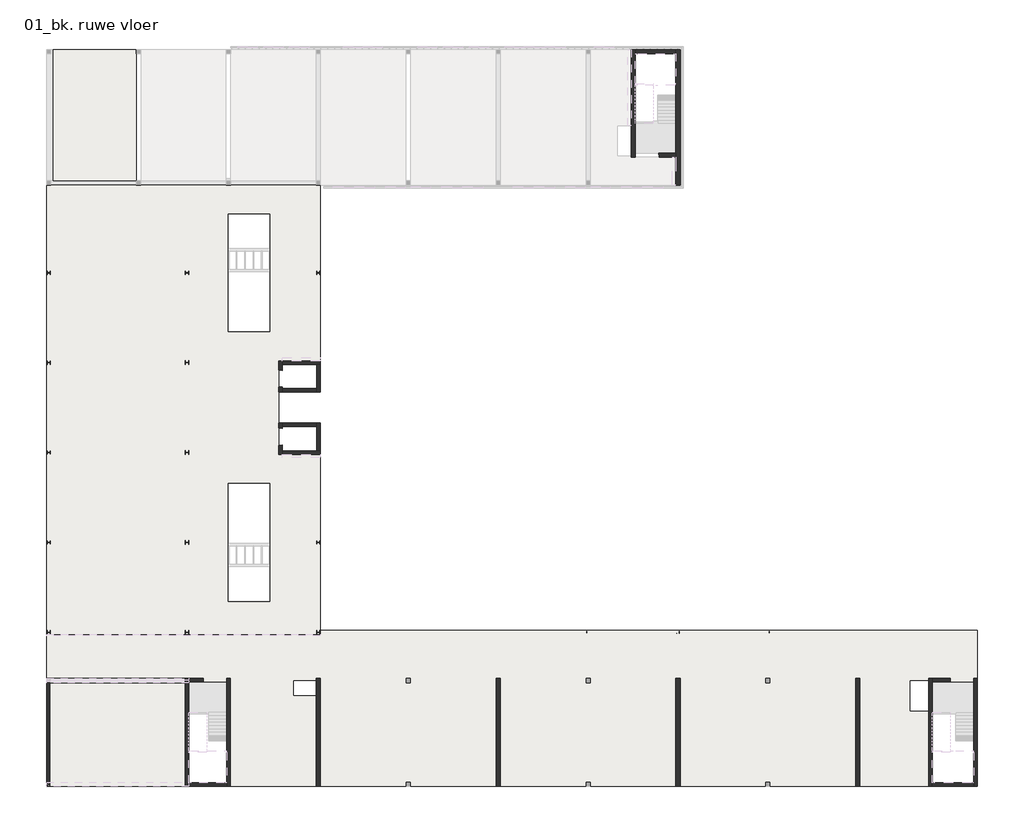
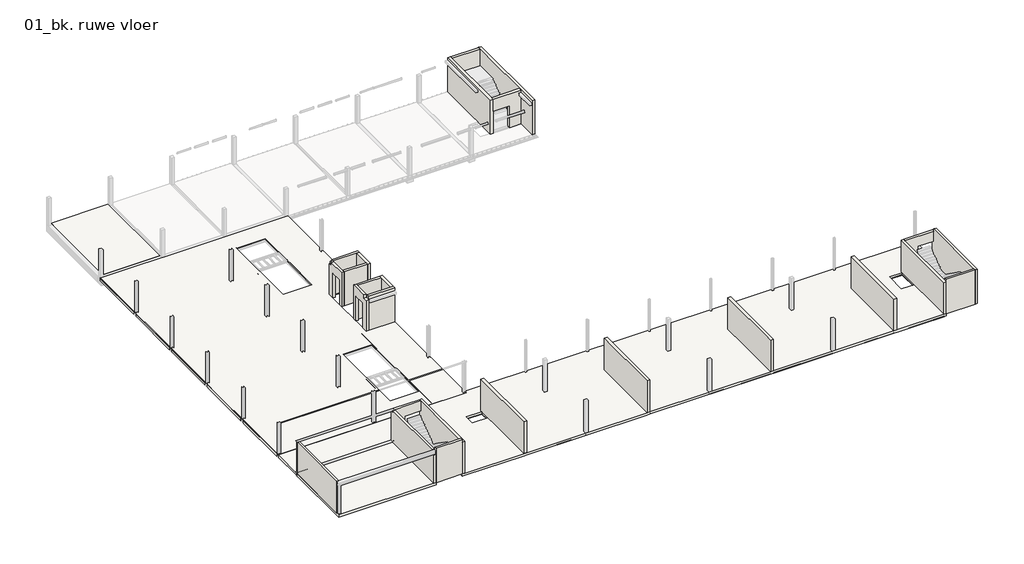
# One storey, part 1 of 4: 25 walls, 20 slabs.
"""IFC4 building model written with IfcOpenShell, lengths in millimetres."""

import ifcopenshell
import ifcopenshell.guid

model = None  # the IFC model being written
_history = None  # IfcOwnerHistory: only IFC2X3 demands one
_inside = {}  # id of a spatial element -> (the spatial element, [elements in it])
_under = {}  # id of a project, library or spatial element -> (it, [spatial elements below it])
_declared = {}  # id of a project -> (the project, [libraries it declares])
_typed = {}  # id of a type object -> (the type object, [elements of that type])
_made_of = {}  # id of a material, layer set ... -> (it, [elements and type objects made of it])


def new_model(schema):
    """Start an empty IFC model of exactly this schema.

    Asked for "IFC4X3", IfcOpenShell would pick the latest addendum, in which some entities
    have other attributes; the version numbers below select the first issue.
    IFC2X3 requires an IfcOwnerHistory on every rooted entity: one is made here for all.
    """
    global model, _history
    if schema == "IFC4X3":
        model = ifcopenshell.file(schema_version=(4, 3, 0, 0))
    else:
        model = ifcopenshell.file(schema=schema)
    _inside.clear()
    _under.clear()
    _declared.clear()
    _typed.clear()
    _made_of.clear()
    _history = None
    if model.schema == "IFC2X3":
        org = make("IfcOrganization", Name="unknown")
        user = make(
            "IfcPersonAndOrganization",
            ThePerson=make("IfcPerson", FamilyName="unknown"),
            TheOrganization=org,
        )
        app = make(
            "IfcApplication",
            ApplicationDeveloper=org,
            Version="unknown",
            ApplicationFullName="unknown",
            ApplicationIdentifier="unknown",
        )
        _history = make(
            "IfcOwnerHistory",
            OwningUser=user,
            OwningApplication=app,
            ChangeAction="ADDED",
            CreationDate=0,
        )
    return model


def make(cls, **values):
    """One entity of the class cls with the attributes given. An attribute that is None is left unset."""
    return model.create_entity(
        cls, **{name: value for name, value in values.items() if value is not None}
    )


def rooted(cls, **values):
    """An entity with a GlobalId (a new one), such as an element, a storey or a relation."""
    return make(cls, GlobalId=ifcopenshell.guid.new(), OwnerHistory=_history, **values)


def si_unit(unit_type, name, prefix=None):
    """IfcSIUnit, for example si_unit("LENGTHUNIT", "METRE", prefix="MILLI")."""
    return make("IfcSIUnit", UnitType=unit_type, Prefix=prefix, Name=name)


def assignment(units):
    """IfcUnitAssignment: the units of a project."""
    return None if units is None else make("IfcUnitAssignment", Units=units)


def point(xyz):
    """IfcCartesianPoint."""
    return None if xyz is None else make("IfcCartesianPoint", Coordinates=xyz)


def direction(xyz):
    """IfcDirection."""
    return None if xyz is None else make("IfcDirection", DirectionRatios=xyz)


def frame(location, z_axis=None, x_axis=None):
    """IfcAxis2Placement3D, a coordinate frame: its origin and axes. An axis left out is left unset."""
    return make(
        "IfcAxis2Placement3D",
        Location=point(location),
        Axis=direction(z_axis),
        RefDirection=direction(x_axis),
    )


def origin():
    """The frame at (0, 0, 0) with its axes left unset."""
    return frame((0.0, 0.0, 0.0))


def place(relative_to, where):
    """IfcLocalPlacement: puts the frame where relative to a parent placement (None: the world)."""
    return make(
        "IfcLocalPlacement", PlacementRelTo=relative_to, RelativePlacement=where
    )


def context(
    kind, dimensions, precision=None, world=None, true_north=None, identifier=None
):
    """IfcGeometricRepresentationContext, for example the 3D "Model" context."""
    return make(
        "IfcGeometricRepresentationContext",
        ContextIdentifier=identifier,
        ContextType=kind,
        CoordinateSpaceDimension=dimensions,
        Precision=precision,
        WorldCoordinateSystem=world,
        TrueNorth=true_north,
    )


def project(units=None, contexts=None):
    """IfcProject with its units and contexts."""
    return rooted(
        "IfcProject",
        Name="project",
        RepresentationContexts=contexts,
        UnitsInContext=assignment(units),
    )


def spatial(cls, under=None, at=None, **own):
    """A site, building, storey or space (cls), placed at a placement, below another one or the project."""
    s = rooted(cls, ObjectPlacement=at, **own)
    if under is not None:
        _under.setdefault(under.id(), (under, []))[1].append(s)
    return s


def polyline(points):
    """IfcPolyline through the points."""
    return make("IfcPolyline", Points=[point(p) for p in points])


def outline(outer, holes=None, kind="AREA"):
    """IfcArbitraryClosedProfileDef: a profile drawn as a closed curve; with holes, ...WithVoids."""
    if holes is None:
        return make("IfcArbitraryClosedProfileDef", ProfileType=kind, OuterCurve=outer)
    return make(
        "IfcArbitraryProfileDefWithVoids",
        ProfileType=kind,
        OuterCurve=outer,
        InnerCurves=holes,
    )


def extrude(swept, where, along, depth):
    """IfcExtrudedAreaSolid: the profile swept, set in the frame where, extruded along a direction by depth."""
    return make(
        "IfcExtrudedAreaSolid",
        SweptArea=swept,
        Position=where,
        ExtrudedDirection=direction(along),
        Depth=depth,
    )


def faces_of(points, faces, orient=None, outer=None):
    """IfcFace entities. A face is a list of loops; a loop is a list of indices into points, from 0.

    orient and outer hold one flag for each loop. By default every Orientation is true, the
    first loop of a face is its IfcFaceOuterBound and the others are IfcFaceBound.
    """
    made = []
    for i, loops in enumerate(faces):
        bounds = []
        for j, loop in enumerate(loops):
            is_outer = j == 0 if outer is None else outer[i][j]
            bounds.append(
                make(
                    "IfcFaceOuterBound" if is_outer else "IfcFaceBound",
                    Bound=make("IfcPolyLoop", Polygon=[points[k] for k in loop]),
                    Orientation=True if orient is None else orient[i][j],
                )
            )
        made.append(make("IfcFace", Bounds=bounds))
    return made


def faceted_brep(points, faces, orient=None, outer=None, voids=None):
    """IfcFacetedBrep: a solid bounded by flat faces; with voids (closed shells), ...WithVoids."""
    shared = [point(p) for p in points]
    hull = make("IfcClosedShell", CfsFaces=faces_of(shared, faces, orient, outer))
    if voids is None:
        return make("IfcFacetedBrep", Outer=hull)
    return make(
        "IfcFacetedBrepWithVoids",
        Outer=hull,
        Voids=[
            make(cls, CfsFaces=faces_of(shared, fs, o, b)) for cls, fs, o, b in voids
        ],
    )


def shape(context_of_items, identifier, shape_type, items):
    """IfcShapeRepresentation: the items that make up one representation, for example the "Body"."""
    return make(
        "IfcShapeRepresentation",
        ContextOfItems=context_of_items,
        RepresentationIdentifier=identifier,
        RepresentationType=shape_type,
        Items=items,
    )


def made_of(thing, what):
    """Note that an element or type object is made of a material, layer set ...; save() writes the relation."""
    if what is not None:
        _made_of.setdefault(what.id(), (what, []))[1].append(thing)
    return thing


def element(
    cls,
    number,
    at=None,
    inside=None,
    cuts=None,
    type_object=None,
    material=None,
    context=None,
    identifier="Body",
    shape_type=None,
    held_by="IfcProductDefinitionShape",
    body=None,
    shapes=None,
    **own,
):
    """One element of the class cls, such as IfcWall. Its Tag is "e" and its number.

    at: its placement. inside: the storey or other place that contains it. cuts: it is an
    opening in that element (IfcRelVoidsElement). A single representation is given by context,
    identifier, shape_type and body (its items); several are given by shapes. held_by: the class
    of the entity that holds the representations. save() writes the other relations.
    """
    e = rooted(cls, Tag="e%d" % number, ObjectPlacement=at, **own)
    if body is not None:
        shapes = [shape(context, identifier, shape_type, body)]
    if shapes is not None:
        e.Representation = make(held_by, Representations=shapes)
    if inside is not None:
        _inside.setdefault(inside.id(), (inside, []))[1].append(e)
    if cuts is not None:
        rooted(
            "IfcRelVoidsElement", RelatingBuildingElement=cuts, RelatedOpeningElement=e
        )
    if type_object is not None:
        _typed.setdefault(type_object.id(), (type_object, []))[1].append(e)
    return made_of(e, material)


def aggregate(whole, parts):
    """IfcRelAggregates: a whole, such as a stair, and the parts it consists of."""
    return rooted("IfcRelAggregates", RelatingObject=whole, RelatedObjects=parts)


def save(model, path):
    """Write the relations noted so far, then the file.

    IfcRelAggregates (storeys below a building ...), IfcRelContainedInSpatialStructure (elements
    in a storey), IfcRelDefinesByType, IfcRelAssociatesMaterial and IfcRelDeclares: one each for
    every whole, place, type object, material and project.
    """
    for whole, parts in _under.values():
        aggregate(whole, parts)
    for where, things in _inside.values():
        rooted(
            "IfcRelContainedInSpatialStructure",
            RelatedElements=things,
            RelatingStructure=where,
        )
    for kind, things in _typed.values():
        rooted("IfcRelDefinesByType", RelatedObjects=things, RelatingType=kind)
    for what, things in _made_of.values():
        rooted("IfcRelAssociatesMaterial", RelatedObjects=things, RelatingMaterial=what)
    for by, libraries in _declared.values():
        rooted("IfcRelDeclares", RelatingContext=by, RelatedDefinitions=libraries)
    model.write(path)


model = new_model("IFC4")

# Units and contexts
model_context = context("Model", 3, world=origin())
ifc_project = project(units=[si_unit("LENGTHUNIT", "METRE", prefix="MILLI")], contexts=[model_context])

# Site, building, storey
site = spatial("IfcSite", under=ifc_project)
building = spatial("IfcBuilding", under=site)
storey = spatial("IfcBuildingStorey", under=building, Name="01_bk. ruwe vloer", Elevation=3730.0)

# Slabs
placement = place(None, origin())
element("IfcSlab", 1, ObjectType="NLRS_23_FL_breedplaat 260_gen_rsf", at=placement, inside=storey, context=model_context, shape_type="Brep", body=[
    faceted_brep([(70375.0, -150.0, 3470.0), (70125.0, -150.0, 3470.0), (65200.0, -150.0, 3470.0), (64800.0, -150.0, 3470.0), (52200.0, -150.0, 3470.0), (51800.0, -150.0, 3470.0), (39200.0, -150.0, 3470.0), (38800.0, -150.0, 3470.0), (26200.0, -150.0, 3470.0), (25800.0, -150.0, 3470.0), (19625.0, -150.0, 3470.0), (19375.0, -150.0, 3470.0), (19375.0, 7400.0, 3470.0), (16625.0, 7400.0, 3470.0), (16625.0, 7493.0, 3470.0), (16625.0, 7507.0, 3470.0), (6350.0, 7507.0, 3470.0), (6350.0, 10845.0, 3470.0), (26125.0, 10845.0, 3470.0), (26125.0, 11125.0, 3470.0), (73650.0, 11125.0, 3470.0), (73650.0, 7400.0, 3470.0), (73400.0, 7400.0, 3470.0), (70375.0, 7400.0, 3470.0), (19600.0, 7622.0, 3470.0), (19600.0, -140.0, 3470.0), (25825.0, -140.0, 3470.0), (25825.0, 125.0, 3470.0), (26175.0, 125.0, 3470.0), (26175.0, -140.0, 3470.0), (32375.0, -140.0, 3470.0), (32375.0, 7625.0, 3470.0), (32625.0, 7625.0, 3470.0), (32625.0, -140.0, 3470.0), (38825.0, -140.0, 3470.0), (38825.0, 125.0, 3470.0), (39175.0, 125.0, 3470.0), (39175.0, -140.0, 3470.0), (45375.0, -140.0, 3470.0), (45375.0, 7625.0, 3470.0), (45625.0, 7625.0, 3470.0), (45625.0, -140.0, 3470.0), (51825.0, -140.0, 3470.0), (51825.0, 125.0, 3470.0), (52175.0, 125.0, 3470.0), (52175.0, -140.0, 3470.0), (58375.0, -140.0, 3470.0), (58375.0, 7625.0, 3470.0), (58625.0, 7625.0, 3470.0), (58625.0, -140.0, 3470.0), (64825.0, -140.0, 3470.0), (64825.0, 125.0, 3470.0), (65175.0, 125.0, 3470.0), (65175.0, -140.0, 3470.0), (70150.0, -140.0, 3470.0), (70150.0, 7625.0, 3470.0), (73640.0, 7625.0, 3470.0), (73640.0, 11115.0, 3470.0), (26135.0, 11115.0, 3470.0), (26135.0, 10750.0, 3470.0), (6360.0, 10750.0, 3470.0), (6360.0, 7622.0, 3470.0), (51825.0, 7625.0, 3470.0), (52175.0, 7625.0, 3470.0), (52175.0, 7375.0, 3470.0), (51825.0, 7375.0, 3470.0), (64825.0, 7625.0, 3470.0), (65175.0, 7625.0, 3470.0), (65175.0, 7375.0, 3470.0), (64825.0, 7375.0, 3470.0), (38825.0, 7625.0, 3470.0), (39175.0, 7625.0, 3470.0), (39175.0, 7375.0, 3470.0), (38825.0, 7375.0, 3470.0), (25850.0, 7375.0, 3470.0), (25850.0, 7500.0, 3470.0), (25825.0, 7500.0, 3470.0), (25825.0, 7625.0, 3470.0), (26175.0, 7625.0, 3470.0), (26175.0, 7375.0, 3470.0), (19375.0, -150.0, 3730.0), (19625.0, -150.0, 3730.0), (25850.0, -150.0, 3730.0), (26150.0, -150.0, 3730.0), (32350.0, -150.0, 3730.0), (32650.0, -150.0, 3730.0), (38850.0, -150.0, 3730.0), (39150.0, -150.0, 3730.0), (45350.0, -150.0, 3730.0), (45650.0, -150.0, 3730.0), (51850.0, -150.0, 3730.0), (52150.0, -150.0, 3730.0), (58350.0, -150.0, 3730.0), (58650.0, -150.0, 3730.0), (64850.0, -150.0, 3730.0), (65150.0, -150.0, 3730.0), (70125.0, -150.0, 3730.0), (70375.0, -150.0, 3730.0), (70375.0, 7400.0, 3730.0), (71700.0, 7400.0, 3730.0), (73650.0, 7400.0, 3730.0), (73650.0, 11125.0, 3730.0), (26125.0, 11125.0, 3730.0), (26125.0, 10845.0, 3730.0), (6350.0, 10845.0, 3730.0), (6350.0, 7507.0, 3730.0), (16625.0, 7507.0, 3730.0), (16625.0, 7493.0, 3730.0), (16625.0, 7400.0, 3730.0), (19375.0, 7400.0, 3730.0), (19375.0, 100.0, 3730.0), (24227.5, 6452.0, 3730.0), (24227.5, 7500.0, 3730.0), (25850.0, 7500.0, 3730.0), (25850.0, 6452.0, 3730.0), (68805.0, 5320.0, 3730.0), (68805.0, 7500.0, 3730.0), (70125.0, 7500.0, 3730.0), (70125.0, 5320.0, 3730.0), (6350.0, 10845.0, 3680.0), (26125.0, 10845.0, 3680.0), (19600.0, -140.0, 3530.0), (19600.0, 7622.0, 3530.0), (6360.0, 7622.0, 3530.0), (6360.0, 10750.0, 3530.0), (26135.0, 10750.0, 3530.0), (26135.0, 11115.0, 3530.0), (73640.0, 11115.0, 3530.0), (73640.0, 7625.0, 3530.0), (70150.0, 7625.0, 3530.0), (70150.0, -140.0, 3530.0), (65175.0, -140.0, 3530.0), (65175.0, 125.0, 3530.0), (64825.0, 125.0, 3530.0), (64825.0, -140.0, 3530.0), (58625.0, -140.0, 3530.0), (58625.0, 7625.0, 3530.0), (58375.0, 7625.0, 3530.0), (58375.0, -140.0, 3530.0), (52175.0, -140.0, 3530.0), (52175.0, 125.0, 3530.0), (51825.0, 125.0, 3530.0), (51825.0, -140.0, 3530.0), (45625.0, -140.0, 3530.0), (45625.0, 7625.0, 3530.0), (45375.0, 7625.0, 3530.0), (45375.0, -140.0, 3530.0), (39175.0, -140.0, 3530.0), (39175.0, 125.0, 3530.0), (38825.0, 125.0, 3530.0), (38825.0, -140.0, 3530.0), (32625.0, -140.0, 3530.0), (32625.0, 7625.0, 3530.0), (32375.0, 7625.0, 3530.0), (32375.0, -140.0, 3530.0), (26175.0, -140.0, 3530.0), (26175.0, 125.0, 3530.0), (25825.0, 125.0, 3530.0), (25825.0, -140.0, 3530.0), (26175.0, 7625.0, 3530.0), (25825.0, 7625.0, 3530.0), (25825.0, 7500.0, 3530.0), (24227.5, 7500.0, 3530.0), (24227.5, 6452.0, 3530.0), (25850.0, 6452.0, 3530.0), (25850.0, 7375.0, 3530.0), (26175.0, 7375.0, 3530.0), (52175.0, 7625.0, 3530.0), (51825.0, 7625.0, 3530.0), (51825.0, 7375.0, 3530.0), (52175.0, 7375.0, 3530.0), (65175.0, 7625.0, 3530.0), (64825.0, 7625.0, 3530.0), (64825.0, 7375.0, 3530.0), (65175.0, 7375.0, 3530.0), (39175.0, 7625.0, 3530.0), (38825.0, 7625.0, 3530.0), (38825.0, 7375.0, 3530.0), (39175.0, 7375.0, 3530.0), (68805.0, 7500.0, 3530.0), (68805.0, 5320.0, 3530.0), (70125.0, 5320.0, 3530.0), (70125.0, 7500.0, 3530.0)], [[[0, 1, 2, 3, 4, 5, 6, 7, 8, 9, 10, 11, 12, 13, 14, 15, 16, 17, 18, 19, 20, 21, 22, 23], [24, 25, 26, 27, 28, 29, 30, 31, 32, 33, 34, 35, 36, 37, 38, 39, 40, 41, 42, 43, 44, 45, 46, 47, 48, 49, 50, 51, 52, 53, 54, 55, 56, 57, 58, 59, 60, 61]], [[62, 63, 64, 65]], [[66, 67, 68, 69]], [[70, 71, 72, 73]], [[74, 75, 76, 77, 78, 79]], [[80, 81, 82, 83, 84, 85, 86, 87, 88, 89, 90, 91, 92, 93, 94, 95, 96, 97, 98, 99, 100, 101, 102, 103, 104, 105, 106, 107, 108, 109, 110], [111, 112, 113, 114], [115, 116, 117, 118]], [[11, 10, 9, 8, 7, 6, 5, 4, 3, 2, 1, 0, 97, 96, 95, 94, 93, 92, 91, 90, 89, 88, 87, 86, 85, 84, 83, 82, 81, 80]], [[12, 11, 80, 110, 109]], [[13, 12, 109, 108]], [[13, 108, 107, 106, 15, 14]], [[17, 16, 105, 104, 119]], [[18, 17, 119, 104, 103, 120]], [[19, 18, 120, 103, 102]], [[20, 19, 102, 101]], [[21, 20, 101, 100]], [[23, 22, 21, 100, 99, 98]], [[0, 23, 98, 97]], [[16, 15, 106, 105]], [[121, 122, 123, 124, 125, 126, 127, 128, 129, 130, 131, 132, 133, 134, 135, 136, 137, 138, 139, 140, 141, 142, 143, 144, 145, 146, 147, 148, 149, 150, 151, 152, 153, 154, 155, 156, 157, 158], [159, 160, 161, 162, 163, 164, 165, 166], [167, 168, 169, 170], [171, 172, 173, 174], [175, 176, 177, 178], [179, 180, 181, 182]], [[122, 121, 25, 24]], [[123, 122, 24, 61]], [[124, 123, 61, 60]], [[125, 124, 60, 59]], [[126, 125, 59, 58]], [[127, 126, 58, 57]], [[128, 127, 57, 56]], [[129, 128, 56, 55]], [[130, 129, 55, 54]], [[131, 130, 54, 53]], [[132, 131, 53, 52]], [[133, 132, 52, 51]], [[134, 133, 51, 50]], [[135, 134, 50, 49]], [[136, 135, 49, 48]], [[137, 136, 48, 47]], [[138, 137, 47, 46]], [[139, 138, 46, 45]], [[140, 139, 45, 44]], [[141, 140, 44, 43]], [[142, 141, 43, 42]], [[143, 142, 42, 41]], [[144, 143, 41, 40]], [[145, 144, 40, 39]], [[146, 145, 39, 38]], [[147, 146, 38, 37]], [[148, 147, 37, 36]], [[149, 148, 36, 35]], [[150, 149, 35, 34]], [[151, 150, 34, 33]], [[152, 151, 33, 32]], [[153, 152, 32, 31]], [[154, 153, 31, 30]], [[155, 154, 30, 29]], [[156, 155, 29, 28]], [[157, 156, 28, 27]], [[158, 157, 27, 26]], [[121, 158, 26, 25]], [[160, 159, 78, 77]], [[161, 160, 77, 76]], [[166, 165, 74, 79]], [[159, 166, 79, 78]], [[168, 167, 63, 62]], [[169, 168, 62, 65]], [[170, 169, 65, 64]], [[167, 170, 64, 63]], [[172, 171, 67, 66]], [[173, 172, 66, 69]], [[174, 173, 69, 68]], [[171, 174, 68, 67]], [[176, 175, 71, 70]], [[177, 176, 70, 73]], [[178, 177, 73, 72]], [[175, 178, 72, 71]], [[112, 111, 163, 162]], [[111, 114, 164, 163]], [[113, 75, 74, 165, 164, 114]], [[75, 113, 112, 162, 161, 76]], [[116, 115, 180, 179]], [[115, 118, 181, 180]], [[118, 117, 182, 181]], [[117, 116, 179, 182]]]),
])
element("IfcSlab", 2, ObjectType="NLRS_23_FL_breedplaat 260_gen_rsf", at=placement, inside=storey, context=model_context, shape_type="Brep", body=[
    faceted_brep([(6830.0, 43680.0, 3470.0), (6830.0, 43800.0, 3470.0), (6830.0, 53150.0, 3470.0), (6950.0, 53150.0, 3470.0), (12700.0, 53150.0, 3470.0), (12820.0, 53150.0, 3470.0), (12820.0, 43680.0, 3470.0), (12700.0, 43680.0, 3470.0), (12725.0, 43775.0, 3470.0), (12725.0, 53140.0, 3470.0), (6925.0, 53140.0, 3470.0), (6925.0, 43775.0, 3470.0), (6830.0, 53150.0, 3730.0), (6830.0, 43680.0, 3730.0), (12820.0, 43680.0, 3730.0), (12820.0, 53150.0, 3730.0), (6925.0, 53140.0, 3530.0), (12725.0, 53140.0, 3530.0), (12725.0, 43775.0, 3530.0), (6925.0, 43775.0, 3530.0)], [[[0, 1, 2, 3, 4, 5, 6, 7], [8, 9, 10, 11]], [[12, 13, 14, 15]], [[2, 1, 0, 13, 12]], [[5, 4, 3, 2, 12, 15]], [[6, 5, 15, 14]], [[0, 7, 6, 14, 13]], [[16, 17, 18, 19]], [[18, 17, 9, 8]], [[19, 18, 8, 11]], [[16, 19, 11, 10]], [[17, 16, 10, 9]]]),
])
element("IfcSlab", 3, ObjectType="NLRS_23_FL_druklaag 70_gen_rsf", at=placement, inside=storey, context=model_context, shape_type="Brep", body=[
    faceted_brep([(26125.0, 23875.0, 3660.0), (26125.0, 23795.0, 3660.0), (26125.0, 17675.0, 3660.0), (26125.0, 17655.0, 3660.0), (26125.0, 17345.0, 3660.0), (26125.0, 17325.0, 3660.0), (26125.0, 11175.0, 3660.0), (26125.0, 11155.0, 3660.0), (6350.0, 11155.0, 3660.0), (6350.0, 11175.0, 3660.0), (6350.0, 17325.0, 3660.0), (6350.0, 17345.0, 3660.0), (19240.0, 17345.0, 3660.0), (19240.0, 17655.0, 3660.0), (6350.0, 17655.0, 3660.0), (6350.0, 17675.0, 3660.0), (6350.0, 23825.0, 3660.0), (6350.0, 23845.0, 3660.0), (19240.0, 23845.0, 3660.0), (19500.0, 23845.0, 3660.0), (22500.0, 23845.0, 3660.0), (22760.0, 23845.0, 3660.0), (23362.3, 23845.0, 3660.0), (23362.3, 23875.0, 3660.0), (22500.0, 21750.0, 3660.0), (19500.0, 21750.0, 3660.0), (19500.0, 13250.0, 3660.0), (22500.0, 13250.0, 3660.0), (19500.0000006, 22062.0, 3660.0), (19500.0000006, 21760.0, 3660.0), (22499.9999994, 21760.0, 3660.0), (22499.9999994, 22062.0, 3660.0), (19500.0000006, 13240.0, 3660.0), (19500.0000006, 12938.0, 3660.0), (22499.9999994, 12938.0, 3660.0), (22499.9999994, 13240.0, 3660.0), (23125.0, 24155.0, 3660.0), (6350.0, 24155.0, 3660.0), (6350.0, 24175.0, 3660.0), (6350.0, 30302.0, 3660.0), (6350.0, 30322.0, 3660.0), (23125.0, 30322.0, 3660.0), (23125.0, 30302.0, 3660.0), (23125.0, 24175.0, 3660.0), (6350.0, 43350.0, 3660.0), (26125.0, 43350.0, 3660.0), (26125.0, 43330.0, 3660.0), (26125.0, 37175.0, 3660.0), (26125.0, 37155.0, 3660.0), (22760.0, 37155.0, 3660.0), (22760.0, 36845.0, 3660.0), (26125.0, 36845.0, 3660.0), (26125.0, 36825.0, 3660.0), (26125.0, 30705.0, 3660.0), (26125.0, 30625.0, 3660.0), (23362.3, 30625.0, 3660.0), (23362.3, 30632.0, 3660.0), (6350.0, 30632.0, 3660.0), (6350.0, 30652.0, 3660.0), (6350.0, 36825.0, 3660.0), (6350.0, 36845.0, 3660.0), (19240.0, 36845.0, 3660.0), (19240.0, 37155.0, 3660.0), (6350.0, 37155.0, 3660.0), (6350.0, 37175.0, 3660.0), (6350.0, 43330.0, 3660.0), (22500.0, 32750.0, 3660.0), (22500.0, 41250.0, 3660.0), (19500.0, 41250.0, 3660.0), (19500.0, 32750.0, 3660.0), (19500.0000006, 41562.0, 3660.0), (19500.0000006, 41260.0, 3660.0), (22499.9999994, 41260.0, 3660.0), (22499.9999994, 41562.0, 3660.0), (19500.0000006, 32740.0, 3660.0), (19500.0000006, 32438.0, 3660.0), (22499.9999994, 32438.0, 3660.0), (22499.9999994, 32740.0, 3660.0), (26125.0, 30625.0, 3730.0), (26125.0, 43350.0, 3730.0), (13180.0, 43350.0, 3730.0), (12820.0, 43350.0, 3730.0), (6350.0, 43350.0, 3730.0), (6350.0, 10845.0, 3730.0), (26125.0, 10845.0, 3730.0), (26125.0, 11125.0, 3730.0), (26125.0, 23875.0, 3730.0), (23125.0, 23875.0, 3730.0), (23125.0, 30625.0, 3730.0), (22500.0, 41250.0, 3730.0), (22500.0, 32750.0, 3730.0), (19500.0, 32750.0, 3730.0), (19500.0, 41250.0, 3730.0), (19500.0, 21750.0, 3730.0), (22500.0, 21750.0, 3730.0), (22500.0, 13250.0, 3730.0), (19500.0, 13250.0, 3730.0), (26125.0, 36845.0, 3680.0), (26125.0, 37155.0, 3680.0), (6350.0, 10845.0, 3680.0), (26125.0, 10845.0, 3680.0), (6350.0, 37155.0, 3680.0), (6350.0, 36845.0, 3680.0), (6350.0, 30632.0, 3680.0), (6350.0, 30322.0, 3680.0), (6350.0, 24155.0, 3680.0), (6350.0, 23845.0, 3680.0), (6350.0, 17655.0, 3680.0), (6350.0, 17345.0, 3680.0), (6350.0, 11155.0, 3680.0), (23125.0, 30625.0, 3680.0), (23362.3, 30625.0, 3680.0), (23125.0, 23875.0, 3680.0), (23125.0, 24155.0, 3680.0), (23125.0, 30322.0, 3680.0), (23362.3, 23875.0, 3680.0), (26125.0, 11125.0, 3680.0), (26125.0, 11155.0, 3680.0), (19240.0, 17345.0, 3680.0), (19240.0, 17655.0, 3680.0), (23362.3, 23845.0, 3680.0), (23362.3, 30632.0, 3680.0), (19240.0, 36845.0, 3680.0), (19240.0, 37155.0, 3680.0), (22760.0, 37155.0, 3680.0), (22760.0, 36845.0, 3680.0), (19500.0000006, 41562.0, 3680.0), (19500.0000006, 41260.0, 3680.0), (22499.9999994, 41260.0, 3680.0), (22499.9999994, 41562.0, 3680.0), (19500.0000006, 32740.0, 3680.0), (19500.0000006, 32438.0, 3680.0), (22499.9999994, 32438.0, 3680.0), (22499.9999994, 32740.0, 3680.0), (19500.0000006, 22062.0, 3680.0), (19500.0000006, 21760.0, 3680.0), (22499.9999994, 21760.0, 3680.0), (22499.9999994, 22062.0, 3680.0), (19500.0000006, 13240.0, 3680.0), (19500.0000006, 12938.0, 3680.0), (22499.9999994, 12938.0, 3680.0), (22499.9999994, 13240.0, 3680.0)], [[[0, 1, 2, 3, 4, 5, 6, 7, 8, 9, 10, 11, 12, 13, 14, 15, 16, 17, 18, 19, 20, 21, 22, 23], [24, 25, 26, 27], [28, 29, 30, 31], [32, 33, 34, 35]], [[36, 37, 38, 39, 40, 41, 42, 43]], [[44, 45, 46, 47, 48, 49, 50, 51, 52, 53, 54, 55, 56, 57, 58, 59, 60, 61, 62, 63, 64, 65], [66, 67, 68, 69], [70, 71, 72, 73], [74, 75, 76, 77]], [[78, 79, 80, 81, 82, 83, 84, 85, 86, 87, 88], [89, 90, 91, 92], [93, 94, 95, 96]], [[79, 78, 54, 53, 52, 51, 97, 98, 48, 47, 46, 45]], [[84, 83, 99, 100]], [[83, 82, 44, 65, 64, 63, 101, 102, 60, 59, 58, 57, 103, 104, 40, 39, 38, 37, 105, 106, 17, 16, 15, 14, 107, 108, 11, 10, 9, 8, 109, 99]], [[45, 44, 82, 81, 80, 79]], [[78, 88, 110, 111, 55, 54]], [[88, 87, 112, 113, 36, 43, 42, 41, 114, 110]], [[87, 86, 0, 23, 115, 112]], [[0, 86, 85, 84, 100, 116, 117, 7, 6, 5, 4, 3, 2, 1]], [[67, 66, 90, 89]], [[68, 67, 89, 92]], [[69, 68, 92, 91]], [[66, 69, 91, 90]], [[25, 24, 94, 93]], [[26, 25, 93, 96]], [[27, 26, 96, 95]], [[24, 27, 95, 94]], [[109, 117, 116, 100, 99]], [[117, 109, 8, 7]], [[118, 119, 13, 12]], [[119, 118, 108, 107]], [[119, 107, 14, 13]], [[108, 118, 12, 11]], [[120, 115, 23, 22]], [[120, 106, 105, 113, 112, 115]], [[113, 105, 37, 36]], [[106, 120, 22, 21, 20, 19, 18, 17]], [[111, 121, 56, 55]], [[103, 121, 111, 110, 114, 104]], [[121, 103, 57, 56]], [[104, 114, 41, 40]], [[122, 123, 62, 61]], [[123, 122, 102, 101]], [[123, 101, 63, 62]], [[102, 122, 61, 60]], [[124, 125, 50, 49]], [[125, 124, 98, 97]], [[98, 124, 49, 48]], [[125, 97, 51, 50]], [[126, 127, 71, 70]], [[128, 129, 73, 72]], [[127, 126, 129, 128]], [[127, 128, 72, 71]], [[129, 126, 70, 73]], [[130, 131, 75, 74]], [[132, 133, 77, 76]], [[131, 130, 133, 132]], [[133, 130, 74, 77]], [[131, 132, 76, 75]], [[134, 135, 29, 28]], [[136, 137, 31, 30]], [[135, 134, 137, 136]], [[135, 136, 30, 29]], [[137, 134, 28, 31]], [[138, 139, 33, 32]], [[140, 141, 35, 34]], [[139, 138, 141, 140]], [[141, 138, 32, 35]], [[139, 140, 34, 33]]]),
])
element("IfcSlab", 4, ObjectType="NLRS_23_FL_kanaalplaat 260_gen_rsf", at=placement, inside=storey, context=model_context, shape_type="SweptSolid", body=[
    extrude(outline(polyline([(19240.0, 11175.0), (6350.0, 11175.0), (6350.0, 17325.0), (19240.0, 17325.0), (19240.0, 11175.0)])), frame((0.0, 0.0, 3400.0), z_axis=(0.0, 0.0, 1.0), x_axis=(1.0, 0.0, 0.0)), (0.0, 0.0, 1.0), 260.0),
])
element("IfcSlab", 5, ObjectType="NLRS_23_FL_kanaalplaat 260_gen_rsf", at=placement, inside=storey, context=model_context, shape_type="SweptSolid", body=[
    extrude(outline(polyline([(6350.0, 17675.0), (6350.0, 23825.0), (19240.0, 23825.0), (19240.0, 17675.0), (6350.0, 17675.0)])), frame((0.0, 0.0, 3400.0), z_axis=(0.0, 0.0, 1.0), x_axis=(1.0, 0.0, 0.0)), (0.0, 0.0, 1.0), 260.0),
])
element("IfcSlab", 6, ObjectType="NLRS_23_FL_kanaalplaat 260_gen_rsf", at=placement, inside=storey, context=model_context, shape_type="SweptSolid", body=[
    extrude(outline(polyline([(23125.0, 30302.0), (23125.0, 24175.0), (6350.0, 24175.0), (6350.0, 30302.0), (23125.0, 30302.0)])), frame((0.0, 0.0, 3400.0), z_axis=(0.0, 0.0, 1.0), x_axis=(1.0, 0.0, 0.0)), (0.0, 0.0, 1.0), 260.0),
])
element("IfcSlab", 7, ObjectType="NLRS_23_FL_kanaalplaat 260_gen_rsf", at=placement, inside=storey, context=model_context, shape_type="SweptSolid", body=[
    extrude(outline(polyline([(22500.0, 23825.0), (22500.0, 22082.0), (19500.0, 22082.0), (19500.0, 23825.0), (22500.0, 23825.0)])), frame((0.0, 0.0, 3400.0), z_axis=(0.0, 0.0, 1.0), x_axis=(1.0, 0.0, 0.0)), (0.0, 0.0, 1.0), 260.0),
])
element("IfcSlab", 8, ObjectType="NLRS_23_FL_kanaalplaat 260_gen_rsf", at=placement, inside=storey, context=model_context, shape_type="SweptSolid", body=[
    extrude(outline(polyline([(22500.0, 11182.5), (19500.0, 11182.5), (19500.0, 12918.0), (22500.0, 12918.0), (22500.0, 11182.5)])), frame((0.0, 0.0, 3400.0), z_axis=(0.0, 0.0, 1.0), x_axis=(1.0, 0.0, 0.0)), (0.0, 0.0, 1.0), 260.0),
])
element("IfcSlab", 9, ObjectType="NLRS_23_FL_kanaalplaat 260_gen_rsf", at=placement, inside=storey, context=model_context, shape_type="Brep", body=[
    faceted_brep([(26125.0, 23795.0, 3400.0), (26125.0, 23625.0, 3400.0), (26125.0, 17675.0, 3400.0), (22760.0, 17675.0, 3400.0), (22760.0, 23825.0, 3400.0), (23395.0, 23825.0, 3400.0), (23395.0, 23795.0, 3400.0), (26125.0, 23795.0, 3660.0), (23395.0, 23795.0, 3660.0), (23395.0, 23825.0, 3660.0), (22760.0, 23825.0, 3660.0), (22760.0, 17675.0, 3660.0), (26125.0, 17675.0, 3660.0)], [[[0, 1, 2, 3, 4, 5, 6]], [[7, 8, 9, 10, 11, 12]], [[2, 1, 0, 7, 12]], [[3, 2, 12, 11]], [[4, 3, 11, 10]], [[5, 4, 10, 9]], [[6, 5, 9, 8]], [[0, 6, 8, 7]]]),
])
element("IfcSlab", 10, ObjectType="NLRS_23_FL_kanaalplaat 260_gen_rsf", at=placement, inside=storey, context=model_context, shape_type="SweptSolid", body=[
    extrude(outline(polyline([(22760.0, 11175.0), (22760.0, 17325.0), (26125.0, 17325.0), (26125.0, 11175.0), (22760.0, 11175.0)])), frame((0.0, 0.0, 3400.0), z_axis=(0.0, 0.0, 1.0), x_axis=(1.0, 0.0, 0.0)), (0.0, 0.0, 1.0), 260.0),
])
element("IfcSlab", 11, ObjectType="NLRS_23_FL_kanaalplaat 260_gen_rsf", at=placement, inside=storey, context=model_context, shape_type="Brep", body=[
    faceted_brep([(19240.0, 43330.0, 3400.0), (19240.0, 37175.0, 3400.0), (6350.0, 37175.0, 3400.0), (6350.0, 43200.0, 3400.0), (6350.0, 43330.0, 3400.0), (19240.0, 43330.0, 3660.0), (6350.0, 43330.0, 3660.0), (6350.0, 37175.0, 3660.0), (19240.0, 37175.0, 3660.0)], [[[0, 1, 2, 3, 4]], [[5, 6, 7, 8]], [[0, 4, 6, 5]], [[4, 3, 2, 7, 6]], [[2, 1, 8, 7]], [[1, 0, 5, 8]]]),
])
element("IfcSlab", 12, ObjectType="NLRS_23_FL_kanaalplaat 260_gen_rsf", at=placement, inside=storey, context=model_context, shape_type="SweptSolid", body=[
    extrude(outline(polyline([(6350.0, 36825.0), (19240.0, 36825.0), (19240.0, 30652.0), (6350.0, 30652.0), (6350.0, 36825.0)])), frame((0.0, 0.0, 3400.0), z_axis=(0.0, 0.0, 1.0), x_axis=(1.0, 0.0, 0.0)), (0.0, 0.0, 1.0), 260.0),
])
element("IfcSlab", 13, ObjectType="NLRS_23_FL_kanaalplaat 260_gen_rsf", at=placement, inside=storey, context=model_context, shape_type="SweptSolid", body=[
    extrude(outline(polyline([(22500.0, 30652.0), (19500.0, 30652.0), (19500.0, 32418.0), (22500.0, 32418.0), (22500.0, 30652.0)])), frame((0.0, 0.0, 3400.0), z_axis=(0.0, 0.0, 1.0), x_axis=(1.0, 0.0, 0.0)), (0.0, 0.0, 1.0), 260.0),
])
element("IfcSlab", 14, ObjectType="NLRS_23_FL_kanaalplaat 260_gen_rsf", at=placement, inside=storey, context=model_context, shape_type="SweptSolid", body=[
    extrude(outline(polyline([(22500.0, 43330.0), (22500.0, 41582.0), (19500.0, 41582.0), (19500.0, 43330.0), (22500.0, 43330.0)])), frame((0.0, 0.0, 3400.0), z_axis=(0.0, 0.0, 1.0), x_axis=(1.0, 0.0, 0.0)), (0.0, 0.0, 1.0), 260.0),
])
element("IfcSlab", 15, ObjectType="NLRS_23_FL_kanaalplaat 260_gen_rsf", at=placement, inside=storey, context=model_context, shape_type="Brep", body=[
    faceted_brep([(26125.0, 30705.0, 3400.0), (23395.0, 30705.0, 3400.0), (23395.0, 30652.0, 3400.0), (22760.0, 30652.0, 3400.0), (22760.0, 36825.0, 3400.0), (26125.0, 36825.0, 3400.0), (26125.0, 30875.0, 3400.0), (26125.0, 30705.0, 3660.0), (26125.0, 36825.0, 3660.0), (22760.0, 36825.0, 3660.0), (22760.0, 30652.0, 3660.0), (23395.0, 30652.0, 3660.0), (23395.0, 30705.0, 3660.0)], [[[0, 1, 2, 3, 4, 5, 6]], [[7, 8, 9, 10, 11, 12]], [[0, 6, 5, 8, 7]], [[5, 4, 9, 8]], [[4, 3, 10, 9]], [[3, 2, 11, 10]], [[2, 1, 12, 11]], [[1, 0, 7, 12]]]),
])
element("IfcSlab", 16, ObjectType="NLRS_23_FL_kanaalplaat 260_gen_rsf", at=placement, inside=storey, context=model_context, shape_type="Brep", body=[
    faceted_brep([(22760.0, 43330.0, 3400.0), (26125.0, 43330.0, 3400.0), (26125.0, 43200.0, 3400.0), (26125.0, 37175.0, 3400.0), (22760.0, 37175.0, 3400.0), (22760.0, 43330.0, 3660.0), (22760.0, 37175.0, 3660.0), (26125.0, 37175.0, 3660.0), (26125.0, 43330.0, 3660.0)], [[[0, 1, 2, 3, 4]], [[5, 6, 7, 8]], [[0, 4, 6, 5]], [[4, 3, 7, 6]], [[3, 2, 1, 8, 7]], [[1, 0, 5, 8]]]),
])
element("IfcSlab", 17, ObjectType="NLRS_23_FL_breedplaat 260_gen_rsf", at=placement, inside=storey, context=model_context, shape_type="Brep", body=[
    faceted_brep([(6350.0, -150.0, 3470.0), (6350.0, 7493.0, 3470.0), (16625.0, 7493.0, 3470.0), (16625.0, -150.0, 3470.0), (6539.0, 125.0, 3470.0), (16400.0, 125.0, 3470.0), (16400.0, 7378.0, 3470.0), (6539.0, 7378.0, 3470.0), (6350.0, 7493.0, 3730.0), (6350.0, -150.0, 3730.0), (16375.0, -150.0, 3730.0), (16625.0, -150.0, 3730.0), (16625.0, 100.0, 3730.0), (16625.0, 7493.0, 3730.0), (16400.0, 7378.0, 3530.0), (16400.0, 125.0, 3530.0), (6539.0, 125.0, 3530.0), (6539.0, 7378.0, 3530.0)], [[[0, 1, 2, 3], [4, 5, 6, 7]], [[8, 9, 10, 11, 12, 13]], [[1, 0, 9, 8]], [[2, 1, 8, 13]], [[3, 2, 13, 12, 11]], [[0, 3, 11, 10, 9]], [[14, 15, 16, 17]], [[16, 15, 5, 4]], [[17, 16, 4, 7]], [[14, 17, 7, 6]], [[15, 14, 6, 5]]]),
])
element("IfcSlab", 18, ObjectType="NLRS_23_FL_breedplaat schil 60_gen_rsf", at=placement, inside=storey, context=model_context, shape_type="SweptSolid", body=[
    extrude(outline(polyline([(16400.0, 125.0), (6539.0, 125.0), (6539.0, 7378.0), (16400.0, 7378.0), (16400.0, 125.0)])), frame((0.0, 0.0, 3470.0), z_axis=(0.0, 0.0, 1.0), x_axis=(1.0, 0.0, 0.0)), (0.0, 0.0, 1.0), 60.0),
])
element("IfcSlab", 19, ObjectType="NLRS_23_FL_breedplaat schil 60_gen_rsf", at=placement, inside=storey, context=model_context, shape_type="SweptSolid", body=[
    extrude(outline(polyline([(19600.0, -140.0), (19600.0, 7622.0), (6360.0, 7622.0), (6360.0, 10750.0), (26135.0, 10750.0), (26135.0, 11115.0), (73640.0, 11115.0), (73640.0, 7625.0), (70150.0, 7625.0), (70150.0, -140.0), (65175.0, -140.0), (65175.0, 125.0), (64825.0, 125.0), (64825.0, -140.0), (58625.0, -140.0), (58625.0, 7625.0), (58375.0, 7625.0), (58375.0, -140.0), (52175.0, -140.0), (52175.0, 125.0), (51825.0, 125.0), (51825.0, -140.0), (45625.0, -140.0), (45625.0, 7625.0), (45375.0, 7625.0), (45375.0, -140.0), (39175.0, -140.0), (39175.0, 125.0), (38825.0, 125.0), (38825.0, -140.0), (32625.0, -140.0), (32625.0, 7625.0), (32375.0, 7625.0), (32375.0, -140.0), (26175.0, -140.0), (26175.0, 125.0), (25825.0, 125.0), (25825.0, -140.0), (19600.0, -140.0)]), holes=[polyline([(26175.0, 7625.0), (25825.0, 7625.0), (25825.0, 7500.0), (24227.5, 7500.0), (24227.5, 6452.0), (25850.0, 6452.0), (25850.0, 7375.0), (26175.0, 7375.0), (26175.0, 7625.0)]), polyline([(52175.0, 7625.0), (51825.0, 7625.0), (51825.0, 7375.0), (52175.0, 7375.0), (52175.0, 7625.0)]), polyline([(65175.0, 7625.0), (64825.0, 7625.0), (64825.0, 7375.0), (65175.0, 7375.0), (65175.0, 7625.0)]), polyline([(39175.0, 7625.0), (38825.0, 7625.0), (38825.0, 7375.0), (39175.0, 7375.0), (39175.0, 7625.0)]), polyline([(68805.0, 7500.0), (68805.0, 5320.0), (70125.0, 5320.0), (70125.0, 7500.0), (68805.0, 7500.0)])]), frame((0.0, 0.0, 3470.0), z_axis=(0.0, 0.0, 1.0), x_axis=(1.0, 0.0, 0.0)), (0.0, 0.0, 1.0), 60.0),
])
element("IfcSlab", 20, ObjectType="NLRS_23_FL_breedplaat schil 60_gen_rsf", at=placement, inside=storey, context=model_context, shape_type="SweptSolid", body=[
    extrude(outline(polyline([(12725.0, 53140.0), (12725.0, 43775.0), (6925.0, 43775.0), (6925.0, 53140.0), (12725.0, 53140.0)])), frame((0.0, 0.0, 3470.0), z_axis=(0.0, 0.0, 1.0), x_axis=(1.0, 0.0, 0.0)), (0.0, 0.0, 1.0), 60.0),
])

# Walls
element("IfcWall", 21, ObjectType="NLRS_22_WA_beton ihw 250_gen_rsf", at=placement, inside=storey, context=model_context, shape_type="Brep", body=[
    faceted_brep([(19625.0, -150.0, 3730.0), (19625.0, 7650.0, 3730.0), (19625.0, 7650.0, 7270.0), (19625.0, -150.0, 7270.0), (19375.0, -150.0, 3730.0), (19375.0, -150.0, 7270.0), (19375.0, 7400.0, 7270.0), (19375.0, 7650.0, 7270.0), (19375.0, 7650.0, 6170.0), (19375.0, 7650.0, 3730.0), (19375.0, 7400.0, 3730.0), (19375.0, 100.0, 3730.0)], [[[0, 1, 2, 3]], [[4, 5, 6, 7, 8, 9, 10, 11]], [[1, 0, 4, 11, 10, 9]], [[2, 1, 9, 8, 7]], [[3, 2, 7, 6, 5]], [[0, 3, 5, 4]]]),
])
element("IfcWall", 22, ObjectType="NLRS_22_WA_beton ihw 250_gen_rsf", at=placement, inside=storey, context=model_context, shape_type="Brep", body=[
    faceted_brep([(16625.0, -150.0, 3730.0), (16625.0, 100.0, 3730.0), (16625.0, 7400.0, 3730.0), (16625.0, 7493.0, 3730.0), (16625.0, 7650.0, 3730.0), (16625.0, 7650.0, 7120.0), (16625.0, 7330.0, 7120.0), (16625.0, 7330.0, 7270.0), (16625.0, 170.0, 7270.0), (16625.0, 170.0, 6880.0), (16625.0, -150.0, 6880.0), (16375.0, -150.0, 3730.0), (16375.0, -150.0, 6880.0), (16375.0, 170.0, 6880.0), (16375.0, 170.0, 7270.0), (16375.0, 7330.0, 7270.0), (16375.0, 7330.0, 7120.0), (16375.0, 7650.0, 7120.0), (16375.0, 7650.0, 3730.0)], [[[0, 1, 2, 3, 4, 5, 6, 7, 8, 9, 10]], [[11, 12, 13, 14, 15, 16, 17, 18]], [[4, 3, 2, 1, 0, 11, 18]], [[5, 4, 18, 17]], [[8, 7, 15, 14]], [[0, 10, 12, 11]], [[6, 5, 17, 16]], [[7, 6, 16, 15]], [[9, 8, 14, 13]], [[10, 9, 13, 12]]]),
])
element("IfcWall", 23, ObjectType="NLRS_22_WA_beton ihw 300_gen_rsf", at=placement, inside=storey, context=model_context, shape_type="Brep", body=[
    faceted_brep([(26150.0, -150.0, 3730.0), (26150.0, 7650.0, 3730.0), (26150.0, 7650.0, 7270.0), (26150.0, -150.0, 7270.0), (25850.0, -150.0, 3730.0), (25850.0, -150.0, 7270.0), (25850.0, 7650.0, 7270.0), (25850.0, 7650.0, 3730.0), (25850.0, 7500.0, 3730.0), (25850.0, 6452.0, 3730.0)], [[[0, 1, 2, 3]], [[4, 5, 6, 7, 8, 9]], [[1, 0, 4, 9, 8, 7]], [[2, 1, 7, 6]], [[3, 2, 6, 5]], [[0, 3, 5, 4]]]),
])
element("IfcWall", 24, ObjectType="NLRS_22_WA_beton ihw 300_gen_rsf", at=placement, inside=storey, context=model_context, shape_type="SweptSolid", body=[
    extrude(outline(polyline([(39150.0, 7650.0), (39150.0, -150.0), (38850.0, -150.0), (38850.0, 7650.0), (39150.0, 7650.0)])), frame((0.0, 0.0, 3730.0), z_axis=(0.0, 0.0, 1.0), x_axis=(1.0, 0.0, 0.0)), (0.0, 0.0, 1.0), 3540.0),
])
element("IfcWall", 25, ObjectType="NLRS_22_WA_beton ihw 300_gen_rsf", at=placement, inside=storey, context=model_context, shape_type="SweptSolid", body=[
    extrude(outline(polyline([(52150.0, 7650.0), (52150.0, -150.0), (51850.0, -150.0), (51850.0, 7650.0), (52150.0, 7650.0)])), frame((0.0, 0.0, 3730.0), z_axis=(0.0, 0.0, 1.0), x_axis=(1.0, 0.0, 0.0)), (0.0, 0.0, 1.0), 3540.0),
])
element("IfcWall", 26, ObjectType="NLRS_22_WA_beton ihw 300_gen_rsf", at=placement, inside=storey, context=model_context, shape_type="SweptSolid", body=[
    extrude(outline(polyline([(65150.0, 7650.0), (65150.0, -150.0), (64850.0, -150.0), (64850.0, 7650.0), (65150.0, 7650.0)])), frame((0.0, 0.0, 3730.0), z_axis=(0.0, 0.0, 1.0), x_axis=(1.0, 0.0, 0.0)), (0.0, 0.0, 1.0), 3540.0),
])
element("IfcWall", 27, ObjectType="NLRS_21_WA_beton ihw 250_gen_rsf", at=placement, inside=storey, context=model_context, shape_type="Brep", body=[
    faceted_brep([(73650.0, -150.0, 3730.0), (73650.0, 7400.0, 3730.0), (73650.0, 7650.0, 3730.0), (73650.0, 7650.0, 7270.0), (73650.0, 7400.0, 7270.0), (73650.0, 7400.0, 7530.0), (73650.0, -150.0, 7530.0), (73400.0, -150.0, 3730.0), (73400.0, -150.0, 7530.0), (73400.0, 100.0, 7530.0), (73400.0, 7400.0, 7530.0), (73400.0, 7400.0, 7270.0), (73400.0, 7650.0, 7270.0), (73400.0, 7650.0, 6170.0), (73400.0, 7650.0, 3730.0), (73400.0, 7400.0, 3730.0), (73400.0, 100.0, 3730.0)], [[[0, 1, 2, 3, 4, 5, 6]], [[7, 8, 9, 10, 11, 12, 13, 14, 15, 16]], [[2, 1, 0, 7, 16, 15, 14]], [[3, 2, 14, 13, 12]], [[6, 5, 10, 9, 8]], [[0, 6, 8, 7]], [[4, 3, 12, 11]], [[5, 4, 11, 10]]]),
])
element("IfcWall", 28, ObjectType="NLRS_21_WA_kalkzandsteen CS12 214_gen_rsf", at=placement, inside=storey, context=model_context, shape_type="SweptSolid", body=[
    extrude(outline(polyline([(6564.0, 7330.0), (6564.0, 170.0), (6350.0, 170.0), (6350.0, 7330.0), (6564.0, 7330.0)])), frame((0.0, 0.0, 3730.0), z_axis=(0.0, 0.0, 1.0), x_axis=(1.0, 0.0, 0.0)), (0.0, 0.0, 1.0), 3540.0),
])
element("IfcWall", 29, ObjectType="NLRS_21_WA_beton ihw 250_gen_rsf", at=placement, inside=storey, context=model_context, shape_type="Brep", body=[
    faceted_brep([(16625.0, -150.0, 3730.0), (19375.0, -150.0, 3730.0), (19375.0, -150.0, 7270.0), (19375.0, -150.0, 7530.0), (16625.0, -150.0, 7530.0), (16625.0, -150.0, 7270.0), (16625.0, -150.0, 6880.0), (19375.0, 100.0, 3730.0), (16625.0, 100.0, 3730.0), (16625.0, 100.0, 7530.0), (19375.0, 100.0, 7530.0), (19375.0, 100.0, 7270.0)], [[[0, 1, 2, 3, 4, 5, 6]], [[7, 8, 9, 10, 11]], [[1, 0, 8, 7]], [[1, 7, 11, 10, 3, 2]], [[4, 3, 10, 9]], [[0, 6, 5, 4, 9, 8]]]),
])
element("IfcWall", 30, ObjectType="NLRS_22_WA_beton ihw 250_gen_rsf", at=placement, inside=storey, context=model_context, shape_type="Brep", body=[
    faceted_brep([(19375.0, 7400.0, 7270.0), (16625.0, 7400.0, 7270.0), (16625.0, 7400.0, 3730.0), (17675.0, 7400.0, 3730.0), (17675.0, 7400.0, 6170.0), (19375.0, 7400.0, 6170.0), (16625.0, 7650.0, 7270.0), (19375.0, 7650.0, 7270.0), (19375.0, 7650.0, 6170.0), (17675.0, 7650.0, 6170.0), (17675.0, 7650.0, 3730.0), (16625.0, 7650.0, 3730.0), (16625.0, 7650.0, 7120.0)], [[[0, 1, 2, 3, 4, 5]], [[6, 7, 8, 9, 10, 11, 12]], [[2, 11, 10, 3]], [[7, 0, 5, 8]], [[1, 0, 7, 6]], [[2, 1, 6, 12, 11]], [[9, 4, 3, 10]], [[4, 9, 8, 5]]]),
])
element("IfcWall", 31, ObjectType="NLRS_22_WA_beton ihw 250_gen_rsf", at=placement, inside=storey, context=model_context, shape_type="Brep", body=[
    faceted_brep([(70375.0, -150.0, 3730.0), (70375.0, 100.0, 3730.0), (70375.0, 7400.0, 3730.0), (70375.0, 7650.0, 3730.0), (70375.0, 7650.0, 7270.0), (70375.0, 7400.0, 7270.0), (70375.0, -150.0, 7270.0), (70125.0, -150.0, 3730.0), (70125.0, -150.0, 7270.0), (70125.0, 7650.0, 7270.0), (70125.0, 7650.0, 3730.0), (70125.0, 7500.0, 3730.0), (70125.0, 5320.0, 3730.0)], [[[0, 1, 2, 3, 4, 5, 6]], [[7, 8, 9, 10, 11, 12]], [[3, 2, 1, 0, 7, 12, 11, 10]], [[4, 3, 10, 9]], [[6, 5, 4, 9, 8]], [[0, 6, 8, 7]]]),
])
element("IfcWall", 32, ObjectType="NLRS_21_WA_beton ihw 250_gen_rsf", at=placement, inside=storey, context=model_context, shape_type="Brep", body=[
    faceted_brep([(70375.0, -150.0, 3730.0), (73400.0, -150.0, 3730.0), (73400.0, -150.0, 7530.0), (70375.0, -150.0, 7530.0), (70375.0, -150.0, 7270.0), (70375.0, 100.0, 3730.0), (70375.0, 100.0, 7530.0), (73400.0, 100.0, 7530.0), (73400.0, 100.0, 3730.0)], [[[0, 1, 2, 3, 4]], [[5, 6, 7, 8]], [[1, 0, 5, 8]], [[2, 1, 8, 7]], [[3, 2, 7, 6]], [[0, 4, 3, 6, 5]]]),
])
element("IfcWall", 33, ObjectType="NLRS_22_WA_beton ihw 250_gen_rsf", at=placement, inside=storey, context=model_context, shape_type="SweptSolid", body=[
    extrude(outline(polyline([(7270.0, 73400.0), (7270.0, 70375.0), (3730.0, 70375.0), (3730.0, 71700.0), (6170.0, 71700.0), (6170.0, 73400.0), (7270.0, 73400.0)])), frame((0.0, 7400.0, 0.0), z_axis=(0.0, 1.0, 0.0), x_axis=(0.0, 0.0, 1.0)), (0.0, 0.0, 1.0), 250.0),
])
element("IfcWall", 34, ObjectType="NLRS_22_WA_beton prefab 300_gen_rsf", at=placement, inside=storey, context=model_context, shape_type="Brep", body=[
    faceted_brep([(48905.0, 45350.0, 3750.0), (48905.0, 53150.0, 3750.0), (48905.0, 53150.0, 7530.0), (48905.0, 45350.0, 7530.0), (48605.0, 45350.0, 3750.0), (48605.0, 45350.0, 7530.0), (48605.0, 53150.0, 7530.0), (48605.0, 53150.0, 7270.0), (48605.0, 53150.0, 7020.0), (48605.0, 53150.0, 3750.0)], [[[0, 1, 2, 3]], [[4, 5, 6, 7, 8, 9]], [[1, 0, 4, 9]], [[2, 1, 9, 8, 7, 6]], [[3, 2, 6, 5]], [[0, 3, 5, 4]]]),
])
element("IfcWall", 35, ObjectType="NLRS_21_WA_beton prefab 300_gen_rsf", at=placement, inside=storey, context=model_context, shape_type="Brep", body=[
    faceted_brep([(52150.0, 43350.0, 3750.0), (52150.0, 53150.0, 3750.0), (52150.0, 53150.0, 7530.0), (52150.0, 43350.0, 7530.0), (51850.0, 43350.0, 3750.0), (51850.0, 43350.0, 7020.0), (51850.0, 43350.0, 7270.0), (51850.0, 43350.0, 7530.0), (51850.0, 53150.0, 7530.0), (51850.0, 53150.0, 3750.0)], [[[0, 1, 2, 3]], [[4, 5, 6, 7, 8, 9]], [[1, 0, 4, 9]], [[2, 1, 9, 8]], [[3, 2, 8, 7]], [[0, 3, 7, 6, 5, 4]]]),
])
element("IfcWall", 36, ObjectType="NLRS_21_WA_beton prefab 300_gen_rsf", at=placement, inside=storey, context=model_context, shape_type="SweptSolid", body=[
    extrude(outline(polyline([(48925.0, 53150.0), (51830.0, 53150.0), (51830.0, 52850.0), (48925.0, 52850.0), (48925.0, 53150.0)])), frame((0.0, 0.0, 3750.0), z_axis=(0.0, 0.0, 1.0), x_axis=(1.0, 0.0, 0.0)), (0.0, 0.0, 1.0), 3780.0),
])
element("IfcWall", 37, ObjectType="NLRS_22_WA_beton prefab 300_gen_rsf", at=placement, inside=storey, context=model_context, shape_type="Brep", body=[
    faceted_brep([(48925.0, 45650.0, 7530.0), (51830.0, 45650.0, 7530.0), (51830.0, 45650.0, 3750.0), (50625.0, 45650.0, 3750.0), (50625.0, 45650.0, 6170.0), (48925.0, 45650.0, 6170.0), (51830.0, 45350.0, 7530.0), (48925.0, 45350.0, 7530.0), (48925.0, 45350.0, 6200.0), (50655.0, 45350.0, 6200.0), (50655.0, 45350.0, 3750.0), (51830.0, 45350.0, 3750.0)], [[[0, 1, 2, 3, 4, 5]], [[6, 7, 8, 9, 10, 11]], [[2, 11, 10, 3]], [[7, 0, 5, 8]], [[1, 0, 7, 6]], [[2, 1, 6, 11]], [[9, 4, 3, 10]], [[4, 9, 8, 5]]]),
])
element("IfcWall", 38, ObjectType="NLRS_22_WA_beton prefab 250_gen_rsf", at=placement, inside=storey, context=model_context, shape_type="Brep", body=[
    faceted_brep([(26125.0, 30625.0, 3750.0), (23395.0, 30625.0, 3750.0), (23395.0, 30625.0, 6950.0), (23395.0, 30625.0, 7200.0), (23395.0, 30625.0, 7530.0), (26125.0, 30625.0, 7530.0), (26125.0, 30625.0, 7200.0), (26125.0, 30625.0, 6950.0), (26125.0, 30375.0, 3750.0), (26125.0, 30375.0, 7530.0), (23395.0, 30375.0, 7530.0), (23395.0, 30375.0, 3750.0)], [[[0, 1, 2, 3, 4, 5, 6, 7]], [[8, 9, 10, 11]], [[1, 0, 8, 11]], [[4, 3, 2, 1, 11, 10]], [[5, 4, 10, 9]], [[0, 7, 6, 5, 9, 8]]]),
])
element("IfcWall", 39, ObjectType="NLRS_22_WA_beton prefab 250_gen_rsf", at=placement, inside=storey, context=model_context, shape_type="Brep", body=[
    faceted_brep([(23125.0, 28375.0, 3750.0), (23125.0, 28375.0, 7530.0), (23125.0, 30231.5, 7530.0), (23125.0, 30231.5, 7155.0), (23125.0, 30625.0, 7155.0), (23125.0, 30625.0, 3750.0), (23125.0, 29973.0, 3750.0), (23125.0, 29973.0, 6505.0), (23125.0, 28723.0, 6505.0), (23125.0, 28723.0, 3750.0), (23375.0, 28375.0, 7530.0), (23375.0, 28375.0, 3750.0), (23375.0, 28748.0, 3750.0), (23375.0, 28748.0, 6480.0), (23375.0, 29948.0, 6480.0), (23375.0, 29948.0, 3750.0), (23375.0, 30625.0, 3750.0), (23375.0, 30625.0, 7155.0), (23375.0, 30231.5, 7155.0), (23375.0, 30231.5, 7530.0)], [[[0, 1, 2, 3, 4, 5, 6, 7, 8, 9]], [[10, 11, 12, 13, 14, 15, 16, 17, 18, 19]], [[11, 0, 9, 12]], [[5, 16, 15, 6]], [[1, 0, 11, 10]], [[2, 1, 10, 19]], [[5, 4, 17, 16]], [[3, 2, 19, 18]], [[4, 3, 18, 17]], [[14, 7, 6, 15]], [[8, 13, 12, 9]], [[7, 14, 13, 8]]]),
])
element("IfcWall", 40, ObjectType="NLRS_22_WA_beton prefab 250_gen_rsf", at=placement, inside=storey, context=model_context, shape_type="SweptSolid", body=[
    extrude(outline(polyline([(25855.0, 28375.0), (23395.0, 28375.0), (23395.0, 28625.0), (25855.0, 28625.0), (25855.0, 28375.0)])), frame((0.0, 0.0, 3750.0), z_axis=(0.0, 0.0, 1.0), x_axis=(1.0, 0.0, 0.0)), (0.0, 0.0, 1.0), 3780.0),
])
element("IfcWall", 41, ObjectType="NLRS_21_WA_beton prefab 250_gen_rsf", at=placement, inside=storey, context=model_context, shape_type="SweptSolid", body=[
    extrude(outline(polyline([(26125.0, 30355.0), (26125.0, 28375.0), (25875.0, 28375.0), (25875.0, 30355.0), (26125.0, 30355.0)])), frame((0.0, 0.0, 3750.0), z_axis=(0.0, 0.0, 1.0), x_axis=(1.0, 0.0, 0.0)), (0.0, 0.0, 1.0), 3780.0),
])
element("IfcWall", 42, ObjectType="NLRS_22_WA_beton prefab 250_gen_rsf", at=placement, inside=storey, context=model_context, shape_type="SweptSolid", body=[
    extrude(outline(polyline([(23395.0, 26125.0), (25855.0, 26125.0), (25855.0, 25875.0), (23395.0, 25875.0), (23395.0, 26125.0)])), frame((0.0, 0.0, 3750.0), z_axis=(0.0, 0.0, 1.0), x_axis=(1.0, 0.0, 0.0)), (0.0, 0.0, 1.0), 3780.0),
])
element("IfcWall", 43, ObjectType="NLRS_22_WA_beton prefab 250_gen_rsf", at=placement, inside=storey, context=model_context, shape_type="Brep", body=[
    faceted_brep([(23125.0, 23875.0, 3750.0), (23125.0, 23875.0, 7155.0), (23125.0, 24291.5, 7155.0), (23125.0, 24291.5, 7530.0), (23125.0, 26125.0, 7530.0), (23125.0, 26125.0, 3750.0), (23125.0, 25777.0, 3750.0), (23125.0, 25777.0, 6505.0), (23125.0, 24527.0, 6505.0), (23125.0, 24527.0, 3750.0), (23375.0, 23875.0, 7155.0), (23375.0, 23875.0, 3750.0), (23375.0, 24552.0, 3750.0), (23375.0, 24552.0, 6480.0), (23375.0, 25752.0, 6480.0), (23375.0, 25752.0, 3750.0), (23375.0, 26125.0, 3750.0), (23375.0, 26125.0, 7530.0), (23375.0, 24291.5, 7530.0), (23375.0, 24291.5, 7155.0)], [[[0, 1, 2, 3, 4, 5, 6, 7, 8, 9]], [[10, 11, 12, 13, 14, 15, 16, 17, 18, 19]], [[11, 0, 9, 12]], [[5, 16, 15, 6]], [[1, 0, 11, 10]], [[4, 3, 18, 17]], [[5, 4, 17, 16]], [[2, 1, 10, 19]], [[3, 2, 19, 18]], [[14, 7, 6, 15]], [[8, 13, 12, 9]], [[7, 14, 13, 8]]]),
])
element("IfcWall", 44, ObjectType="NLRS_22_WA_beton prefab 250_gen_rsf", at=placement, inside=storey, context=model_context, shape_type="Brep", body=[
    faceted_brep([(23395.0, 23875.0, 3750.0), (26125.0, 23875.0, 3750.0), (26125.0, 23875.0, 6950.0), (26125.0, 23875.0, 7200.0), (26125.0, 23875.0, 7530.0), (23395.0, 23875.0, 7530.0), (23395.0, 23875.0, 7200.0), (23395.0, 23875.0, 6950.0), (23395.0, 24125.0, 3750.0), (23395.0, 24125.0, 7530.0), (26125.0, 24125.0, 7530.0), (26125.0, 24125.0, 3750.0)], [[[0, 1, 2, 3, 4, 5, 6, 7]], [[8, 9, 10, 11]], [[1, 0, 8, 11]], [[4, 3, 2, 1, 11, 10]], [[5, 4, 10, 9]], [[0, 7, 6, 5, 9, 8]]]),
])
element("IfcWall", 45, ObjectType="NLRS_21_WA_beton prefab 250_gen_rsf", at=placement, inside=storey, context=model_context, shape_type="SweptSolid", body=[
    extrude(outline(polyline([(26125.0, 26125.0), (26125.0, 24145.0), (25875.0, 24145.0), (25875.0, 26125.0), (26125.0, 26125.0)])), frame((0.0, 0.0, 3750.0), z_axis=(0.0, 0.0, 1.0), x_axis=(1.0, 0.0, 0.0)), (0.0, 0.0, 1.0), 3780.0),
])

save(model, "model.ifc")

# Revit data of these elements
# Type "NLRS_23_FL_breedplaat 260_gen_rsf"
#   Keynote = ""
#   Type IfcGUID = "2ajLwCSRTE_9I1Spg4tpL_"
#   Type Comments = "d=260mm"
#   Description = "breedplaatvloer, vrijdragend"
#   Assembly Code = "23.21"
#   IfcExportAs = "IfcSlab"
#   Function = 1
#   Layers, outside or top first: 260 mm "NLRS_f2_beton ihwg_gen_rsf" (function 1)
# Type "NLRS_23_FL_druklaag 70_gen_rsf"
#   Keynote = ""
#   Type IfcGUID = "2GRbcre991teoKeCLB8MGP"
#   Type Comments = "d=70mm"
#   Description = "druklaag"
#   Assembly Code = "23.21"
#   IfcExportAs = "IfcSlab"
#   Function = 1
#   Layers, outside or top first: 70 mm "NLRS_f2_beton ihwg_gen_rsf" (function 1)
# Type "NLRS_23_FL_kanaalplaat 260_gen_rsf"
#   Keynote = ""
#   Type IfcGUID = "3PAoVTCyX39AT9TmkNvcbI"
#   Type Comments = "d=260mm"
#   Description = "prefab kanaalplaatvloer, vrijdragend"
#   Assembly Code = "23.21"
#   Type Mark = ""
#   IfcExportAs = "IfcSlab"
#   Function = 0
#   Layers, outside or top first: 35 mm "NLRS_f2_beton prefab_gen_rsf" (function 1); 180 mm "NLRS_f2_beton prefab_gen_rsf" (function 1); 45 mm "NLRS_f2_beton prefab_gen_rsf" (function 1)
# Type "NLRS_23_FL_breedplaat schil 60_gen_rsf"
#   Keynote = ""
#   Type IfcGUID = "3PAoVTCyX39AT9TmkNvccm"
#   Type Comments = "d=60mm"
#   Description = "prefab breedplaatvloer, vrijdragend"
#   Assembly Code = "23.21"
#   Type Mark = ""
#   IfcExportAs = "IfcSlab"
#   Function = 0
#   Layers, outside or top first: 60 mm "NLRS_f2_beton prefab_gen_rsf" (function 1)
# Type "NLRS_22_WA_beton ihw 250_gen_rsf"
#   Keynote = ""
#   Type IfcGUID = "1xcRxxwlX9cP9p3jVIop5v"
#   Description = "buitenwand beton ihw, generiek"
#   Assembly Code = "22.21"
#   IfcExportAs = "IfcWall"
#   Layers, outside or top first: 250 mm "NLRS_f2_beton ihwg_gen_rsf" (function 1)
# Type "NLRS_22_WA_beton ihw 300_gen_rsf"
#   Keynote = ""
#   Type IfcGUID = "2lw04Qbvr9TgC3fLWwYnwo"
#   Description = "binnenwand beton ihw, generiek"
#   Assembly Code = "22.21"
#   IfcExportAs = "IfcWall"
#   Layers, outside or top first: 300 mm "NLRS_f2_beton ihwg_gen_rsf" (function 1)
